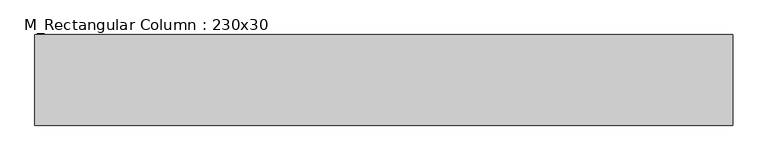
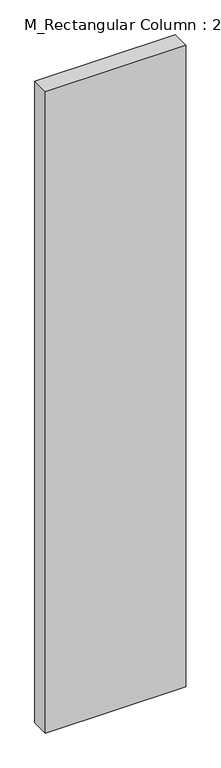
"""IFC4 building model written with IfcOpenShell, lengths in millimetres: column geometry, M_Rectangular Column : 230x30."""

from ifc_helpers import new_model, si_unit, frame, origin, place, context, project, spatial, polyline, outline, extrude, source, transform, mapped, element, save


def m_rectangular_column_230x30_624f9335(model_context):
    return source(origin(), model_context, "Body", "SweptSolid", [
        extrude(outline(polyline([(1150.0, 150.0), (1150.0, -150.0), (-1150.0, -150.0), (-1150.0, 150.0), (1150.0, 150.0)])), frame((0.0, 0.0, -3200.0), z_axis=(0.0, 0.0, 1.0), x_axis=(1.0, 0.0, 0.0)), (0.0, 0.0, 1.0), 11100.0),
    ])


if __name__ == "__main__":
    model = new_model("IFC4")
    model_context = context("Model", 3, world=origin())
    ifc_project = project(units=[si_unit("LENGTHUNIT", "METRE", prefix="MILLI")], contexts=[model_context])
    site = spatial("IfcSite", under=ifc_project)
    building = spatial("IfcBuilding", under=site)
    placement = place(None, origin())
    m_rectangular_column_230x30_shape = m_rectangular_column_230x30_624f9335(model_context)
    element("IfcColumn", 1, ObjectType="M_Rectangular Column : 230x30", at=placement, inside=building, context=model_context, shape_type="MappedRepresentation", body=[
        mapped(m_rectangular_column_230x30_shape, transform((0.0, 0.0, 0.0), x_axis=(1.0, 0.0, 0.0), y_axis=(0.0, 1.0, 0.0), z_axis=(0.0, 0.0, 1.0))),
    ])
    save(model, "model.ifc")

# Revit data of these elements
# Type "M_Rectangular Column : 230x30"
#   Depth = 30 cm
#   Offset Base = 0 cm
#   Offset Top = 0 cm
#   Width = 230 cm
#   Material = none
